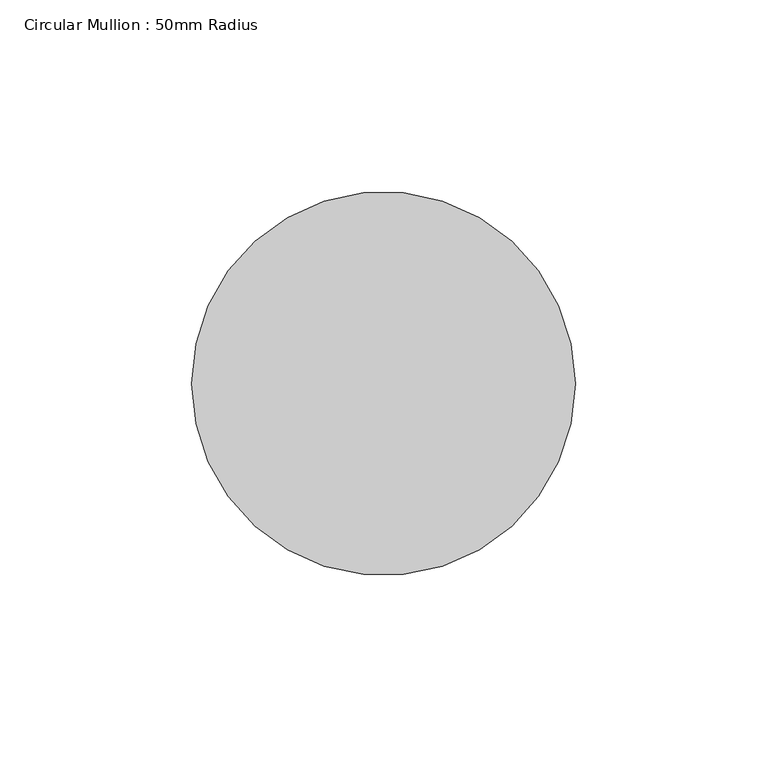
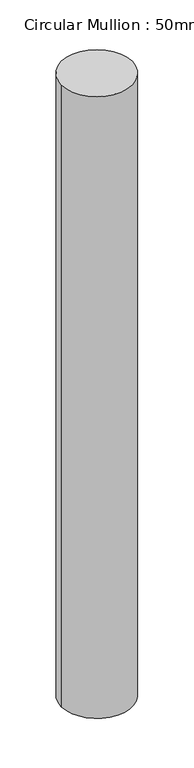
"""IFC4 building model written with IfcOpenShell, lengths in millimetres: member geometry, Circular Mullion : 50mm Radius."""

import ifcopenshell
import ifcopenshell.guid

model = None  # the IFC model being written
_history = None  # IfcOwnerHistory: only IFC2X3 demands one
_inside = {}  # id of a spatial element -> (the spatial element, [elements in it])
_under = {}  # id of a project, library or spatial element -> (it, [spatial elements below it])
_declared = {}  # id of a project -> (the project, [libraries it declares])
_typed = {}  # id of a type object -> (the type object, [elements of that type])
_made_of = {}  # id of a material, layer set ... -> (it, [elements and type objects made of it])


def new_model(schema):
    """Start an empty IFC model of exactly this schema.

    Asked for "IFC4X3", IfcOpenShell would pick the latest addendum, in which some entities
    have other attributes; the version numbers below select the first issue.
    IFC2X3 requires an IfcOwnerHistory on every rooted entity: one is made here for all.
    """
    global model, _history
    if schema == "IFC4X3":
        model = ifcopenshell.file(schema_version=(4, 3, 0, 0))
    else:
        model = ifcopenshell.file(schema=schema)
    _inside.clear()
    _under.clear()
    _declared.clear()
    _typed.clear()
    _made_of.clear()
    _history = None
    if model.schema == "IFC2X3":
        org = make("IfcOrganization", Name="unknown")
        user = make(
            "IfcPersonAndOrganization",
            ThePerson=make("IfcPerson", FamilyName="unknown"),
            TheOrganization=org,
        )
        app = make(
            "IfcApplication",
            ApplicationDeveloper=org,
            Version="unknown",
            ApplicationFullName="unknown",
            ApplicationIdentifier="unknown",
        )
        _history = make(
            "IfcOwnerHistory",
            OwningUser=user,
            OwningApplication=app,
            ChangeAction="ADDED",
            CreationDate=0,
        )
    return model


def make(cls, **values):
    """One entity of the class cls with the attributes given. An attribute that is None is left unset."""
    return model.create_entity(
        cls, **{name: value for name, value in values.items() if value is not None}
    )


def rooted(cls, **values):
    """An entity with a GlobalId (a new one), such as an element, a storey or a relation."""
    return make(cls, GlobalId=ifcopenshell.guid.new(), OwnerHistory=_history, **values)


def si_unit(unit_type, name, prefix=None):
    """IfcSIUnit, for example si_unit("LENGTHUNIT", "METRE", prefix="MILLI")."""
    return make("IfcSIUnit", UnitType=unit_type, Prefix=prefix, Name=name)


def assignment(units):
    """IfcUnitAssignment: the units of a project."""
    return None if units is None else make("IfcUnitAssignment", Units=units)


def point(xyz):
    """IfcCartesianPoint."""
    return None if xyz is None else make("IfcCartesianPoint", Coordinates=xyz)


def direction(xyz):
    """IfcDirection."""
    return None if xyz is None else make("IfcDirection", DirectionRatios=xyz)


def frame(location, z_axis=None, x_axis=None):
    """IfcAxis2Placement3D, a coordinate frame: its origin and axes. An axis left out is left unset."""
    return make(
        "IfcAxis2Placement3D",
        Location=point(location),
        Axis=direction(z_axis),
        RefDirection=direction(x_axis),
    )


def frame_2d(location, x_axis=None):
    """IfcAxis2Placement2D, a coordinate frame in the plane: its origin and x axis."""
    return make(
        "IfcAxis2Placement2D", Location=point(location), RefDirection=direction(x_axis)
    )


def origin():
    """The frame at (0, 0, 0) with its axes left unset."""
    return frame((0.0, 0.0, 0.0))


def origin_2d():
    """The frame at (0, 0) in the plane with its x axis left unset."""
    return frame_2d((0.0, 0.0))


def place(relative_to, where):
    """IfcLocalPlacement: puts the frame where relative to a parent placement (None: the world)."""
    return make(
        "IfcLocalPlacement", PlacementRelTo=relative_to, RelativePlacement=where
    )


def context(
    kind, dimensions, precision=None, world=None, true_north=None, identifier=None
):
    """IfcGeometricRepresentationContext, for example the 3D "Model" context."""
    return make(
        "IfcGeometricRepresentationContext",
        ContextIdentifier=identifier,
        ContextType=kind,
        CoordinateSpaceDimension=dimensions,
        Precision=precision,
        WorldCoordinateSystem=world,
        TrueNorth=true_north,
    )


def project(units=None, contexts=None):
    """IfcProject with its units and contexts."""
    return rooted(
        "IfcProject",
        Name="project",
        RepresentationContexts=contexts,
        UnitsInContext=assignment(units),
    )


def spatial(cls, under=None, at=None, **own):
    """A site, building, storey or space (cls), placed at a placement, below another one or the project."""
    s = rooted(cls, ObjectPlacement=at, **own)
    if under is not None:
        _under.setdefault(under.id(), (under, []))[1].append(s)
    return s


def circle_curve(where, radius):
    """IfcCircle in the frame where."""
    return make("IfcCircle", Position=where, Radius=radius)


def trimmed(basis, trim1, trim2, sense, master):
    """IfcTrimmedCurve: the piece of a basis curve between two trims."""
    return make(
        "IfcTrimmedCurve",
        BasisCurve=basis,
        Trim1=trim1,
        Trim2=trim2,
        SenseAgreement=sense,
        MasterRepresentation=master,
    )


def segment(curve, same_sense, transition):
    """IfcCompositeCurveSegment."""
    return make(
        "IfcCompositeCurveSegment",
        Transition=transition,
        SameSense=same_sense,
        ParentCurve=curve,
    )


def composite_curve(segments, self_intersect=None):
    """IfcCompositeCurve: segments joined end to end."""
    return make("IfcCompositeCurve", Segments=segments, SelfIntersect=self_intersect)


def outline(outer, holes=None, kind="AREA"):
    """IfcArbitraryClosedProfileDef: a profile drawn as a closed curve; with holes, ...WithVoids."""
    if holes is None:
        return make("IfcArbitraryClosedProfileDef", ProfileType=kind, OuterCurve=outer)
    return make(
        "IfcArbitraryProfileDefWithVoids",
        ProfileType=kind,
        OuterCurve=outer,
        InnerCurves=holes,
    )


def extrude(swept, where, along, depth):
    """IfcExtrudedAreaSolid: the profile swept, set in the frame where, extruded along a direction by depth."""
    return make(
        "IfcExtrudedAreaSolid",
        SweptArea=swept,
        Position=where,
        ExtrudedDirection=direction(along),
        Depth=depth,
    )


def shape(context_of_items, identifier, shape_type, items):
    """IfcShapeRepresentation: the items that make up one representation, for example the "Body"."""
    return make(
        "IfcShapeRepresentation",
        ContextOfItems=context_of_items,
        RepresentationIdentifier=identifier,
        RepresentationType=shape_type,
        Items=items,
    )


def source(mapping_origin, context_of_items, identifier, shape_type, items):
    """IfcRepresentationMap: a shape defined once, which mapped items show again and again."""
    return make(
        "IfcRepresentationMap",
        MappingOrigin=mapping_origin,
        MappedRepresentation=shape(context_of_items, identifier, shape_type, items),
    )


def transform(
    local_origin,
    x_axis=None,
    y_axis=None,
    z_axis=None,
    scale=None,
    scale2=None,
    scale3=None,
    uniform=True,
):
    """IfcCartesianTransformationOperator3D, or its non-uniform kind. x_axis, y_axis, z_axis: its Axis1, 2, 3."""
    if uniform:
        return make(
            "IfcCartesianTransformationOperator3D",
            Axis1=direction(x_axis),
            Axis2=direction(y_axis),
            LocalOrigin=point(local_origin),
            Scale=scale,
            Axis3=direction(z_axis),
        )
    return make(
        "IfcCartesianTransformationOperator3DnonUniform",
        Axis1=direction(x_axis),
        Axis2=direction(y_axis),
        LocalOrigin=point(local_origin),
        Scale=scale,
        Axis3=direction(z_axis),
        Scale2=scale2,
        Scale3=scale3,
    )


def mapped(mapping_source, mapping_target):
    """IfcMappedItem: shows the shape of a source again, moved by a transform."""
    return make(
        "IfcMappedItem", MappingSource=mapping_source, MappingTarget=mapping_target
    )


def made_of(thing, what):
    """Note that an element or type object is made of a material, layer set ...; save() writes the relation."""
    if what is not None:
        _made_of.setdefault(what.id(), (what, []))[1].append(thing)
    return thing


def element(
    cls,
    number,
    at=None,
    inside=None,
    cuts=None,
    type_object=None,
    material=None,
    context=None,
    identifier="Body",
    shape_type=None,
    held_by="IfcProductDefinitionShape",
    body=None,
    shapes=None,
    **own,
):
    """One element of the class cls, such as IfcWall. Its Tag is "e" and its number.

    at: its placement. inside: the storey or other place that contains it. cuts: it is an
    opening in that element (IfcRelVoidsElement). A single representation is given by context,
    identifier, shape_type and body (its items); several are given by shapes. held_by: the class
    of the entity that holds the representations. save() writes the other relations.
    """
    e = rooted(cls, Tag="e%d" % number, ObjectPlacement=at, **own)
    if body is not None:
        shapes = [shape(context, identifier, shape_type, body)]
    if shapes is not None:
        e.Representation = make(held_by, Representations=shapes)
    if inside is not None:
        _inside.setdefault(inside.id(), (inside, []))[1].append(e)
    if cuts is not None:
        rooted(
            "IfcRelVoidsElement", RelatingBuildingElement=cuts, RelatedOpeningElement=e
        )
    if type_object is not None:
        _typed.setdefault(type_object.id(), (type_object, []))[1].append(e)
    return made_of(e, material)


def aggregate(whole, parts):
    """IfcRelAggregates: a whole, such as a stair, and the parts it consists of."""
    return rooted("IfcRelAggregates", RelatingObject=whole, RelatedObjects=parts)


def save(model, path):
    """Write the relations noted so far, then the file.

    IfcRelAggregates (storeys below a building ...), IfcRelContainedInSpatialStructure (elements
    in a storey), IfcRelDefinesByType, IfcRelAssociatesMaterial and IfcRelDeclares: one each for
    every whole, place, type object, material and project.
    """
    for whole, parts in _under.values():
        aggregate(whole, parts)
    for where, things in _inside.values():
        rooted(
            "IfcRelContainedInSpatialStructure",
            RelatedElements=things,
            RelatingStructure=where,
        )
    for kind, things in _typed.values():
        rooted("IfcRelDefinesByType", RelatedObjects=things, RelatingType=kind)
    for what, things in _made_of.values():
        rooted("IfcRelAssociatesMaterial", RelatedObjects=things, RelatingMaterial=what)
    for by, libraries in _declared.values():
        rooted("IfcRelDeclares", RelatingContext=by, RelatedDefinitions=libraries)
    model.write(path)


def circular_mullion_50mm_radius_cdf223a6(model_context):
    return source(origin(), model_context, "Body", "SweptSolid", [
        extrude(outline(composite_curve([segment(trimmed(circle_curve(origin_2d(), 50.0), [point((50.0, 0.0))], [point((-50.0, 0.0))], False, "CARTESIAN"), True, "CONTINUOUS"), segment(trimmed(circle_curve(origin_2d(), 50.0), [point((-50.0, 0.0))], [point((50.0, 0.0))], False, "CARTESIAN"), True, "CONTINUOUS")], self_intersect=False)), frame((0.0, 0.0, -925.6368718), z_axis=(0.0, 0.0, 1.0), x_axis=(1.0, 0.0, 0.0)), (0.0, 0.0, 1.0), 925.6368718),
    ])


if __name__ == "__main__":
    model = new_model("IFC4")
    model_context = context("Model", 3, world=origin())
    ifc_project = project(units=[si_unit("LENGTHUNIT", "METRE", prefix="MILLI")], contexts=[model_context])
    site = spatial("IfcSite", under=ifc_project)
    building = spatial("IfcBuilding", under=site)
    placement = place(None, origin())
    circular_mullion_50mm_radius_shape = circular_mullion_50mm_radius_cdf223a6(model_context)
    element("IfcMember", 1, ObjectType="Circular Mullion : 50mm Radius", at=placement, inside=building, context=model_context, shape_type="MappedRepresentation", body=[
        mapped(circular_mullion_50mm_radius_shape, transform((0.0, 0.0, 0.0), x_axis=(1.0, 0.0, 0.0), y_axis=(0.0, 1.0, 0.0), z_axis=(0.0, 0.0, 1.0))),
    ])
    save(model, "model.ifc")

# Revit data of these elements
# Type "Circular Mullion : 50mm Radius"
#   built-in parameter 1007350 = 0.164042 (stored number, unit not read)
# Element 1 (IfcMember, "Circular Mullion : 50mm Radius")
#   Materials on its faces: "Aluminium"
# Materials
#   "Aluminium": class "Metal", colour RGB 247 247 247, transparency 0, Description = "Aluminium 6061", Cost = 0
